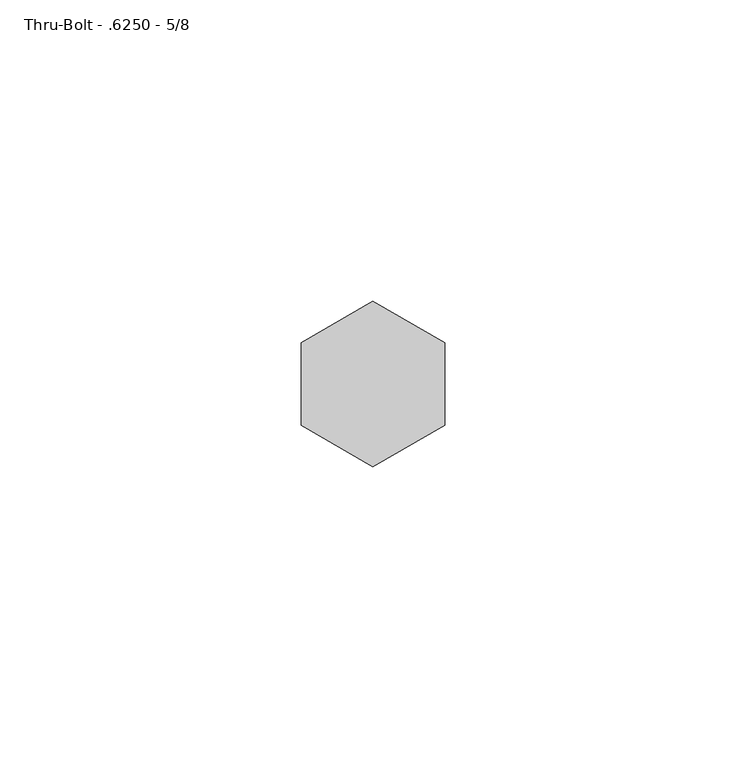
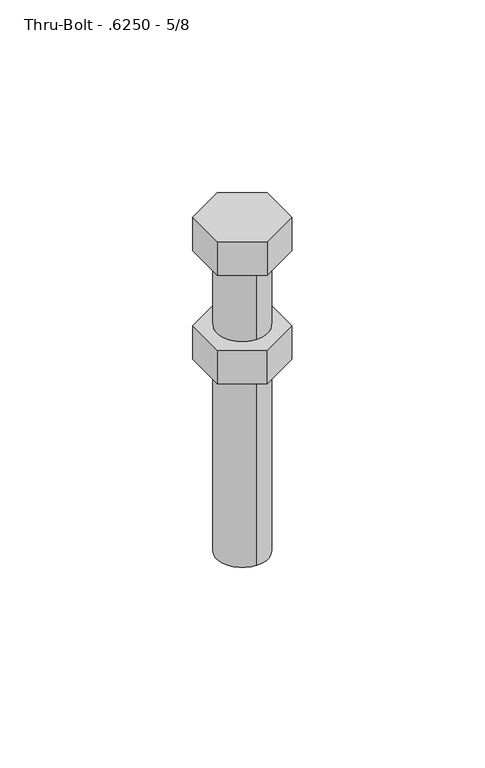
"""IFC4 building model written with IfcOpenShell, lengths in millimetres: fastener geometry, 060523 - W_P_C - Fastenings - Generic : Thru-Bolt - .6250 - 5/8."""

from ifc_helpers import new_model, si_unit, point, frame, origin, origin_with_axes, origin_2d, place, context, project, spatial, polyline, circle_curve, trimmed, segment, composite_curve, outline, extrude, source, transform, mapped, element, save


def thru_bolt_6250_5_8_a49b0b25(model_context):
    return source(origin(), model_context, "Body", "SweptSolid", [
        extrude(outline(polyline([(-11.90625, -6.8740766), (-11.90625, 6.8740766), (0.0, 13.7481533), (11.90625, 6.8740766), (11.90625, -6.8740766), (0.0, -13.7481533), (-11.90625, -6.8740766)])), frame((0.0, 0.0, -36.7109375), z_axis=(0.0, 0.0, 1.0), x_axis=(1.0, 0.0, 0.0)), (0.0, 0.0, 1.0), 11.3109375),
        extrude(outline(polyline([(-11.90625, 6.8740766), (0.0, 13.7481533), (11.90625, 6.8740766), (11.90625, -6.8740766), (0.0, -13.7481533), (-11.90625, -6.8740766), (-11.90625, 6.8740766)])), origin_with_axes(), (0.0, 0.0, 1.0), 11.3109375),
        extrude(outline(composite_curve([segment(trimmed(circle_curve(origin_2d(), 8.1359375), [point((0.0, -8.1359375))], [point((0.0, 8.1359375))], False, "CARTESIAN"), True, "CONTINUOUS"), segment(trimmed(circle_curve(origin_2d(), 8.1359375), [point((0.0, 8.1359375))], [point((0.0, -8.1359375))], False, "CARTESIAN"), True, "CONTINUOUS")], self_intersect=False)), frame((0.0, 0.0, -101.6), z_axis=(0.0, 0.0, 1.0), x_axis=(1.0, 0.0, 0.0)), (0.0, 0.0, 1.0), 101.6),
    ])


if __name__ == "__main__":
    model = new_model("IFC4")
    model_context = context("Model", 3, world=origin())
    ifc_project = project(units=[si_unit("LENGTHUNIT", "METRE", prefix="MILLI")], contexts=[model_context])
    site = spatial("IfcSite", under=ifc_project)
    building = spatial("IfcBuilding", under=site)
    placement = place(None, origin())
    thru_bolt_6250_5_8_shape = thru_bolt_6250_5_8_a49b0b25(model_context)
    element("IfcFastener", 1, ObjectType="060523 - W_P_C - Fastenings - Generic : Thru-Bolt - .6250 - 5/8", at=placement, inside=building, context=model_context, shape_type="MappedRepresentation", body=[
        mapped(thru_bolt_6250_5_8_shape, transform((0.0, 0.0, 0.0), x_axis=(1.0, 0.0, 0.0), y_axis=(0.0, 1.0, 0.0), z_axis=(0.0, 0.0, 1.0))),
    ])
    save(model, "model.ifc")

# Revit data of these elements
# Type "060523 - W_P_C - Fastenings - Generic : Thru-Bolt - .6250 - 5/8"
#   Washer_Thickness = 0' - 0 19/128"
#   Washer Radius = 0' - 0 49/64"
#   Washer Offset - Head = 0' - 0"
#   Washer Offset = 0' - 0"
#   Thickness_of_Substrate [instance default] = 0' - 1"
#   Side = 0' - 0.54199"
#   Radius = 0' - 0 41/128"
#   Length [instance default] = 0' - 4"
#   Head Size = 0' - 0 15/16"
#   Head Radius = 0' - 0 15/32"
#   Head Height = 0' - 0 57/128"
#   Double Diameter = 0' - 1 9/32"
#   Diameter = 0' - 0 41/64"
#   Default Elevation = 4' - 0"
#   Washer_Nut_Visibility = no
#   Washer_Head_Visibility = no
#   Round_Head_Visibility = no
#   Point Visibility = no
#   Nut_Visibility = yes
#   Hex_Head_Visiblilty = yes
#   Washer Material = none
#   Bolt Material (Size) = AT SILL - FASTENER AT 24" O.C.
# Element 1 (IfcFastener, "060523 - W_P_C - Fastenings - Generic : Thru-Bolt - .6250 - 5/8")
#   Materials on its faces: "AT SILL - FASTENER AT 24\" O.C."
# Materials
#   "AT SILL - FASTENER AT 24\" O.C.": class "Generic", colour RGB 120 120 120, transparency 0, Cost = 0
